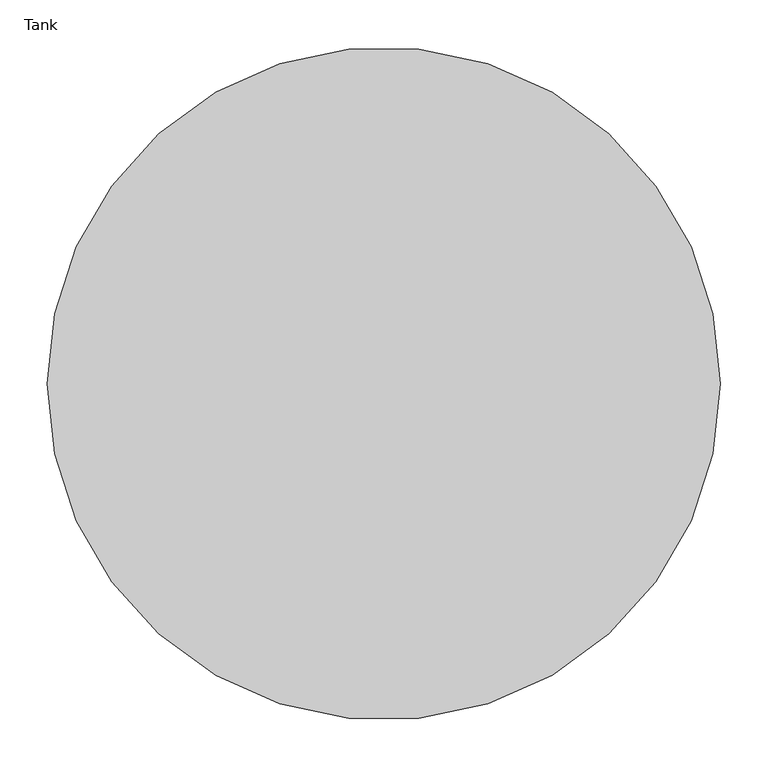
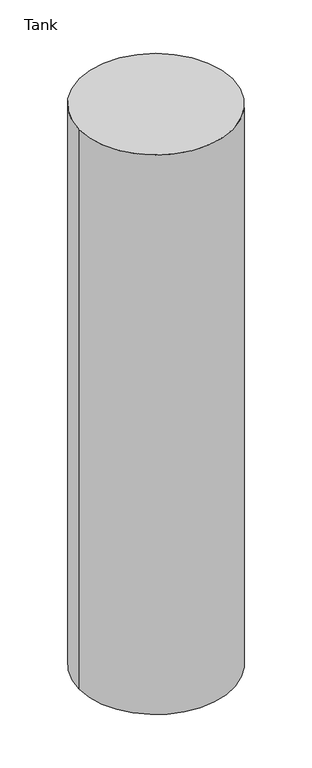
"""IFC4 building model written with IfcOpenShell, lengths in millimetres: proxy geometry, Tank : Brew Kettle."""

from ifc_helpers import new_model, si_unit, point, origin, origin_with_axes, origin_2d, place, context, project, spatial, circle_curve, trimmed, segment, composite_curve, outline, extrude, source, transform, mapped, element, save


def tank_f8dcf229(model_context):
    return source(origin(), model_context, "Body", "SweptSolid", [
        extrude(outline(composite_curve([segment(trimmed(circle_curve(origin_2d(), 355.6), [point((-355.6, 0.0))], [point((355.6, 0.0))], False, "CARTESIAN"), True, "CONTINUOUS"), segment(trimmed(circle_curve(origin_2d(), 355.6), [point((355.6, 0.0))], [point((-355.6, 0.0))], False, "CARTESIAN"), True, "CONTINUOUS")], self_intersect=False)), origin_with_axes(), (0.0, 0.0, 1.0), 2743.2),
    ])


if __name__ == "__main__":
    model = new_model("IFC4")
    model_context = context("Model", 3, world=origin())
    ifc_project = project(units=[si_unit("LENGTHUNIT", "METRE", prefix="MILLI")], contexts=[model_context])
    site = spatial("IfcSite", under=ifc_project)
    building = spatial("IfcBuilding", under=site)
    placement = place(None, origin())
    tank_shape = tank_f8dcf229(model_context)
    element("IfcBuildingElementProxy", 1, Name="Tank : Brew Kettle", ObjectType="Tank : Brew Kettle", at=placement, inside=building, context=model_context, shape_type="MappedRepresentation", body=[
        mapped(tank_shape, transform((0.0, 0.0, 0.0), x_axis=(1.0, 0.0, 0.0), y_axis=(0.0, 1.0, 0.0), z_axis=(0.0, 0.0, 1.0))),
    ])
    save(model, "model.ifc")

# Revit data of these elements
# Type "Tank : Brew Kettle"
#   radius = 1' - 2"
#   Height = 9' - 0"
#   Diameter = 2' - 4"
#   Material = BREW KETTLE
# Element 1 (IfcBuildingElementProxy, "Tank : Brew Kettle")
#   Materials on its faces: "BREW KETTLE"
# Materials
#   "BREW KETTLE": class "Generic", colour RGB 181 181 181, transparency 0, Cost = 0
